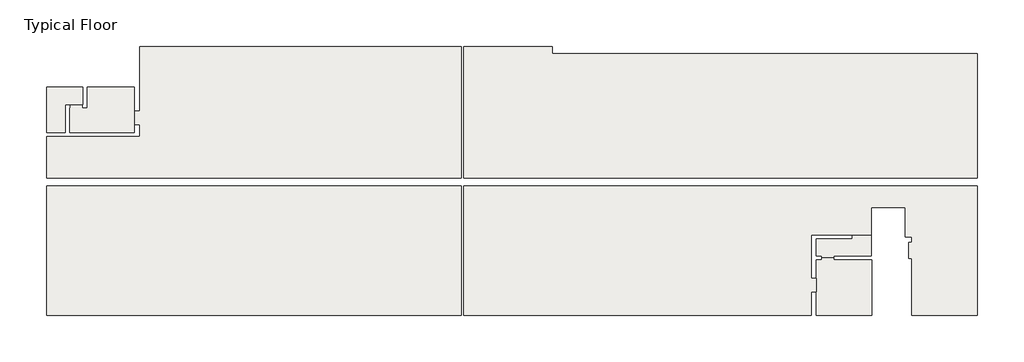
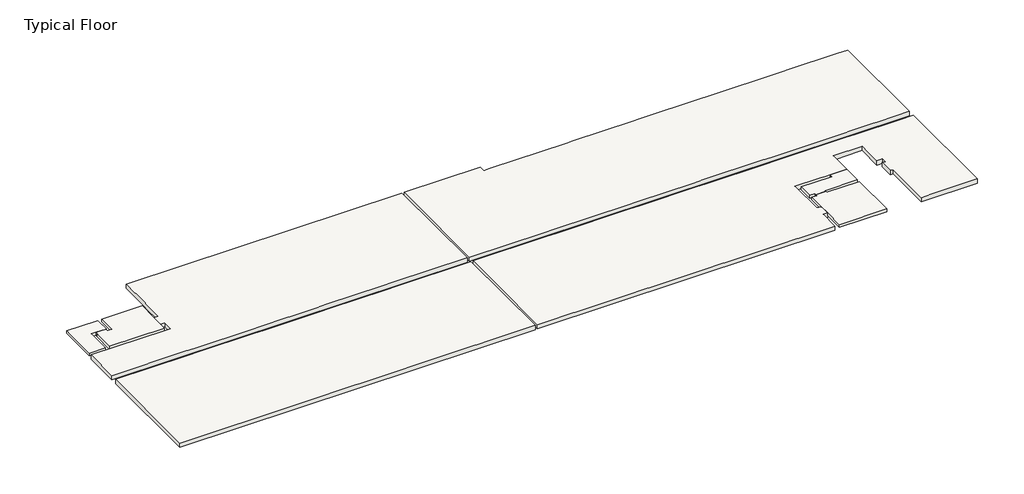
# One storey: 8 slabs.
"""IFC4 building model written with IfcOpenShell, lengths in millimetres."""

from ifc_helpers import new_model, si_unit, frame, origin, place, context, project, spatial, polyline, outline, extrude, faceted_brep, element, save

model = new_model("IFC4")

# Units and contexts
model_context = context("Model", 3, world=origin())
ifc_project = project(units=[si_unit("LENGTHUNIT", "METRE", prefix="MILLI")], contexts=[model_context])

# Site, building, storey
site = spatial("IfcSite", under=ifc_project)
building = spatial("IfcBuilding", under=site)
storey = spatial("IfcBuildingStorey", under=building, Name="Typical Floor", Elevation=4500.0)

# Slabs
placement = place(None, origin())
element("IfcSlab", 1, ObjectType="25", at=placement, inside=storey, context=model_context, shape_type="Brep", body=[
    faceted_brep([(22592.8106957, -3883.3566788, 4250.0), (23037.1054794, -3883.3566788, 4250.0), (23037.1054794, -3733.3566788, 4250.0), (23943.9406174, -3733.3566788, 4250.0), (23943.9406174, -3883.3566788, 4250.0), (26869.9357672, -3883.3566788, 4250.0), (26893.3884, -3883.3566788, 4250.0), (26893.3884, -8183.3289062, 4250.0), (22592.8106957, -8183.3289062, 4250.0), (22592.8106957, -6342.9498143, 4250.0), (23037.1054794, -3883.3566788, 4500.0), (22592.8106957, -3883.3566788, 4500.0), (22592.8106957, -5323.3186801, 4500.0), (22592.8106957, -6342.9498143, 4500.0), (22592.8106957, -8183.3289062, 4500.0), (26893.3884, -8183.3289062, 4500.0), (26893.3884, -3883.3566788, 4500.0), (26869.9357672, -3883.3566788, 4500.0), (23943.9406174, -3883.3566788, 4500.0), (23943.9406174, -3733.3566788, 4500.0), (23037.1054794, -3733.3566788, 4500.0)], [[[0, 1, 2, 3, 4, 5, 6, 7, 8, 9]], [[10, 11, 12, 13, 14, 15, 16, 17, 18, 19, 20]], [[1, 0, 11, 10]], [[2, 1, 10, 20]], [[3, 2, 20, 19]], [[4, 3, 19, 18]], [[4, 18, 17, 16, 6, 5]], [[7, 6, 16, 15]], [[8, 7, 15, 14]], [[9, 8, 14, 13]], [[0, 9, 13, 12, 11]]]),
])
element("IfcSlab", 2, ObjectType="25", at=placement, inside=storey, context=model_context, shape_type="SweptSolid", body=[
    extrude(outline(polyline([(26869.9357672, -1932.7380409), (26869.9357672, -3583.3566788), (23943.9406174, -3583.3566788), (23943.9406174, -3733.3566788), (23037.1054794, -3733.3566788), (23037.1054794, -3583.3566788), (22592.8106957, -3583.3566788), (22592.8106957, -2232.7380409), (25386.8359355, -2232.7380409), (25386.8359355, -1932.7380409), (26869.9357672, -1932.7380409)])), frame((0.0, 0.0, 4250.0), z_axis=(0.0, 0.0, 1.0), x_axis=(1.0, 0.0, 0.0)), (0.0, 0.0, 1.0), 250.0),
])
element("IfcSlab", 3, ObjectType="25", at=placement, inside=storey, context=model_context, shape_type="Brep", body=[
    faceted_brep([(-30180.4573498, 5997.6022486, 4250.0), (-35175.2356133, 5997.6022486, 4250.0), (-35175.2356133, 7897.529186, 4250.0), (-35131.0080225, 7897.529186, 4250.0), (-35131.0080225, 8167.529186, 4250.0), (-34230.8736368, 8167.529186, 4250.0), (-34230.8736368, 7897.529186, 4250.0), (-33829.9452937, 7897.529186, 4250.0), (-33829.9452937, 8167.529186, 4250.0), (-33829.9452937, 9500.978884, 4250.0), (-30180.4573498, 9500.978884, 4250.0), (-30180.4573498, 7652.6880547, 4250.0), (-30180.4573498, 6627.4729602, 4250.0), (-35175.2356133, 5997.6022486, 4500.0), (-30180.4573498, 5997.6022486, 4500.0), (-30180.4573498, 6627.4729602, 4500.0), (-30180.4573498, 7652.6880547, 4500.0), (-30180.4573498, 9500.978884, 4500.0), (-33829.9452937, 9500.978884, 4500.0), (-33829.9452937, 8167.529186, 4500.0), (-33829.9452937, 7897.529186, 4500.0), (-34230.8736368, 7897.529186, 4500.0), (-34230.8736368, 8167.529186, 4500.0), (-35131.0080225, 8167.529186, 4500.0), (-35131.0080225, 7897.529186, 4500.0), (-35175.2356133, 7897.529186, 4500.0)], [[[0, 1, 2, 3, 4, 5, 6, 7, 8, 9, 10, 11, 12]], [[13, 14, 15, 16, 17, 18, 19, 20, 21, 22, 23, 24, 25]], [[1, 0, 14, 13]], [[2, 1, 13, 25]], [[3, 2, 25, 24]], [[4, 3, 24, 23]], [[5, 4, 23, 22]], [[6, 5, 22, 21]], [[7, 6, 21, 20]], [[7, 20, 19, 18, 9, 8]], [[10, 9, 18, 17]], [[10, 17, 16, 15, 14, 0, 12, 11]]]),
])
element("IfcSlab", 4, ObjectType="25", at=placement, inside=storey, context=model_context, shape_type="Brep", body=[
    faceted_brep([(-36981.5324359, 5997.6022486, 4250.0), (-36981.5324359, 9500.978884, 4250.0), (-34179.9452937, 9500.978884, 4250.0), (-34179.9452937, 8167.529186, 4250.0), (-34230.8736368, 8167.529186, 4250.0), (-35131.0080225, 8167.529186, 4250.0), (-35525.2356133, 8167.529186, 4250.0), (-35525.2356133, 7897.529186, 4250.0), (-35525.2356133, 5997.6022486, 4250.0), (-36981.5324359, 9500.978884, 4500.0), (-36981.5324359, 5997.6022486, 4500.0), (-35525.2356133, 5997.6022486, 4500.0), (-35525.2356133, 7897.529186, 4500.0), (-35525.2356133, 8167.529186, 4500.0), (-35131.0080225, 8167.529186, 4500.0), (-34230.8736368, 8167.529186, 4500.0), (-34179.9452937, 8167.529186, 4500.0), (-34179.9452937, 9500.978884, 4500.0)], [[[0, 1, 2, 3, 4, 5, 6, 7, 8]], [[9, 10, 11, 12, 13, 14, 15, 16, 17]], [[1, 0, 10, 9]], [[2, 1, 9, 17]], [[3, 2, 17, 16]], [[3, 16, 15, 14, 13, 6, 5, 4]], [[6, 13, 12, 11, 8, 7]], [[0, 8, 11, 10]]]),
])
element("IfcSlab", 5, ObjectType="40", at=placement, inside=storey, context=model_context, shape_type="Brep", body=[
    faceted_brep([(-4686.1401685, 1852.6133039, 4100.0), (35073.6352373, 1852.6133039, 4100.0), (35073.6352373, -8183.3289062, 4100.0), (29994.7199004, -8183.3289062, 4100.0), (29994.7199004, -3766.5105737, 4100.0), (29744.7199004, -3766.5105737, 4100.0), (29744.7199004, -2514.5866947, 4100.0), (29994.7199004, -2514.5866947, 4100.0), (29994.7199004, -2110.3079756, 4100.0), (29744.7199004, -2110.3079756, 4100.0), (29495.5138576, -2110.3079756, 4100.0), (29495.5138576, 189.1668387, 4100.0), (29245.5138576, 189.1668387, 4100.0), (27139.9357672, 189.1668387, 4100.0), (26869.9357672, 189.1668387, 4100.0), (26869.9357672, -1932.7380409, 4100.0), (25386.8359355, -1932.7380409, 4100.0), (22592.8106957, -1932.7380409, 4100.0), (22192.8106957, -1932.7380409, 4100.0), (22192.8106957, -5323.3186801, 4100.0), (22592.8106957, -5323.3186801, 4100.0), (22592.8106957, -6342.9498143, 4100.0), (22192.8106957, -6342.9498143, 4100.0), (22192.8106957, -8183.3289062, 4100.0), (-4686.1401685, -8183.3289062, 4100.0), (35073.6352373, 1852.6133039, 4500.0), (34927.3208435, 1852.6133039, 4500.0), (34027.3208435, 1852.6133039, 4500.0), (29920.3049975, 1852.6133039, 4500.0), (29020.3049975, 1852.6133039, 4500.0), (22627.3114752, 1852.6133039, 4500.0), (21727.3114752, 1852.6133039, 4500.0), (16420.7293524, 1852.6133039, 4500.0), (15520.7293524, 1852.6133039, 4500.0), (10422.0355776, 1852.6133039, 4500.0), (9522.0355776, 1852.6133039, 4500.0), (2924.3455353, 1852.6133039, 4500.0), (2024.3455353, 1852.6133039, 4500.0), (-4686.1401685, 1852.6133039, 4500.0), (-4686.1401685, -8183.3289062, 4500.0), (22192.8106957, -8183.3289062, 4500.0), (22192.8106957, -6342.9498143, 4500.0), (22592.8106957, -6342.9498143, 4500.0), (22592.8106957, -5323.3186801, 4500.0), (22192.8106957, -5323.3186801, 4500.0), (22192.8106957, -1932.7380409, 4500.0), (22592.8106957, -1932.7380409, 4500.0), (25386.8359355, -1932.7380409, 4500.0), (26869.9357672, -1932.7380409, 4500.0), (26869.9357672, 189.1668387, 4500.0), (27139.9357672, 189.1668387, 4500.0), (29245.5138576, 189.1668387, 4500.0), (29495.5138576, 189.1668387, 4500.0), (29495.5138576, -2110.3079756, 4500.0), (29744.7199004, -2110.3079756, 4500.0), (29994.7199004, -2110.3079756, 4500.0), (29994.7199004, -2514.5866947, 4500.0), (29744.7199004, -2514.5866947, 4500.0), (29744.7199004, -3766.5105737, 4500.0), (29994.7199004, -3766.5105737, 4500.0), (29994.7199004, -8183.3289062, 4500.0), (30873.6352373, -8183.3289062, 4500.0), (35073.6352373, -8183.3289062, 4500.0), (26869.9357672, -1932.7380409, 4250.0), (25386.8359355, -1932.7380409, 4250.0), (22592.8106957, -5323.3186801, 4250.0), (22592.8106957, -6342.9498143, 4250.0)], [[[0, 1, 2, 3, 4, 5, 6, 7, 8, 9, 10, 11, 12, 13, 14, 15, 16, 17, 18, 19, 20, 21, 22, 23, 24]], [[25, 26, 27, 28, 29, 30, 31, 32, 33, 34, 35, 36, 37, 38, 39, 40, 41, 42, 43, 44, 45, 46, 47, 48, 49, 50, 51, 52, 53, 54, 55, 56, 57, 58, 59, 60, 61, 62]], [[1, 0, 38, 37, 36, 35, 34, 33, 32, 31, 30, 29, 28, 27, 26, 25]], [[2, 1, 25, 62]], [[3, 2, 62, 61, 60]], [[4, 3, 60, 59]], [[5, 4, 59, 58]], [[6, 5, 58, 57]], [[7, 6, 57, 56]], [[8, 7, 56, 55]], [[8, 55, 54, 53, 10, 9]], [[11, 10, 53, 52]], [[11, 52, 51, 50, 49, 14, 13, 12]], [[15, 14, 49, 48, 63]], [[16, 15, 63, 48, 47, 64]], [[45, 18, 17, 16, 64, 47, 46]], [[19, 18, 45, 44]], [[20, 19, 44, 43, 65]], [[21, 20, 65, 43, 42, 66]], [[22, 21, 66, 42, 41]], [[23, 22, 41, 40]], [[24, 23, 40, 39]], [[0, 24, 39, 38]]]),
])
element("IfcSlab", 6, ObjectType="40", at=placement, inside=storey, context=model_context, shape_type="Brep", body=[
    faceted_brep([(-4886.1401685, 1852.6133039, 4100.0), (-4886.1401685, -8183.3289062, 4100.0), (-36981.5324359, -8183.3289062, 4100.0), (-36981.5324359, 1852.6133039, 4100.0), (-4886.1401685, 1852.6133039, 4500.0), (-11589.7528998, 1852.6133039, 4500.0), (-12489.7528998, 1852.6133039, 4500.0), (-17591.3777818, 1852.6133039, 4500.0), (-18491.3777818, 1852.6133039, 4500.0), (-23534.5891488, 1852.6133039, 4500.0), (-24434.5891488, 1852.6133039, 4500.0), (-29484.6297539, 1852.6133039, 4500.0), (-30384.6297539, 1852.6133039, 4500.0), (-36981.5324359, 1852.6133039, 4500.0), (-36981.5324359, -8183.3289062, 4500.0), (-4886.1401685, -8183.3289062, 4500.0)], [[[0, 1, 2, 3]], [[4, 5, 6, 7, 8, 9, 10, 11, 12, 13, 14, 15]], [[1, 0, 4, 15]], [[2, 1, 15, 14]], [[3, 2, 14, 13]], [[0, 3, 13, 12, 11, 10, 9, 8, 7, 6, 5, 4]]]),
])
element("IfcSlab", 7, ObjectType="40", at=placement, inside=storey, context=model_context, shape_type="Brep", body=[
    faceted_brep([(2174.3455353, 12665.9833477, 4100.0), (2174.3455353, 12115.9833477, 4100.0), (2774.3455353, 12115.9833477, 4100.0), (9672.0355776, 12115.9833477, 4100.0), (10272.0355776, 12115.9833477, 4100.0), (15670.7293524, 12115.9833477, 4100.0), (16270.7293524, 12115.9833477, 4100.0), (21877.3114752, 12115.9833477, 4100.0), (22477.3114752, 12115.9833477, 4100.0), (29170.3049975, 12115.9833477, 4100.0), (29770.3049975, 12115.9833477, 4100.0), (34177.3208435, 12115.9833477, 4100.0), (34777.3208435, 12115.9833477, 4100.0), (35073.6352373, 12115.9833477, 4100.0), (35073.6352373, 2452.6133039, 4100.0), (-4686.1401685, 2452.6133039, 4100.0), (-4686.1401685, 12665.9833477, 4100.0), (2174.3455353, 12115.9833477, 4500.0), (2174.3455353, 12665.9833477, 4500.0), (-4686.1401685, 12665.9833477, 4500.0), (-4686.1401685, 2452.6133039, 4500.0), (2024.3455353, 2452.6133039, 4500.0), (2924.3455353, 2452.6133039, 4500.0), (9522.0355776, 2452.6133039, 4500.0), (10422.0355776, 2452.6133039, 4500.0), (15520.7293524, 2452.6133039, 4500.0), (16420.7293524, 2452.6133039, 4500.0), (21727.3114752, 2452.6133039, 4500.0), (22627.3114752, 2452.6133039, 4500.0), (29020.3049975, 2452.6133039, 4500.0), (29920.3049975, 2452.6133039, 4500.0), (34027.3208435, 2452.6133039, 4500.0), (34927.3208435, 2452.6133039, 4500.0), (35073.6352373, 2452.6133039, 4500.0), (35073.6352373, 12115.9833477, 4500.0), (34777.3208435, 12115.9833477, 4500.0), (34177.3208435, 12115.9833477, 4500.0), (29770.3049975, 12115.9833477, 4500.0), (29170.3049975, 12115.9833477, 4500.0), (22477.3114752, 12115.9833477, 4500.0), (21877.3114752, 12115.9833477, 4500.0), (16270.7293524, 12115.9833477, 4500.0), (15670.7293524, 12115.9833477, 4500.0), (10272.0355776, 12115.9833477, 4500.0), (9672.0355776, 12115.9833477, 4500.0), (2774.3455353, 12115.9833477, 4500.0)], [[[0, 1, 2, 3, 4, 5, 6, 7, 8, 9, 10, 11, 12, 13, 14, 15, 16]], [[17, 18, 19, 20, 21, 22, 23, 24, 25, 26, 27, 28, 29, 30, 31, 32, 33, 34, 35, 36, 37, 38, 39, 40, 41, 42, 43, 44, 45]], [[1, 0, 18, 17]], [[1, 17, 45, 44, 43, 42, 41, 40, 39, 38, 37, 36, 35, 34, 13, 12, 11, 10, 9, 8, 7, 6, 5, 4, 3, 2]], [[14, 13, 34, 33]], [[15, 14, 33, 32, 31, 30, 29, 28, 27, 26, 25, 24, 23, 22, 21, 20]], [[16, 15, 20, 19]], [[0, 16, 19, 18]]]),
])
element("IfcSlab", 8, ObjectType="40", at=placement, inside=storey, context=model_context, shape_type="Brep", body=[
    faceted_brep([(-29780.4573498, 5697.6022486, 4100.0), (-29780.4573498, 6627.4729602, 4100.0), (-30180.4573498, 6627.4729602, 4100.0), (-30180.4573498, 7652.6880547, 4100.0), (-29780.4573498, 7652.6880547, 4100.0), (-29780.4573498, 9500.978884, 4100.0), (-29780.4573498, 9800.978884, 4100.0), (-29780.4573498, 12665.9833477, 4100.0), (-4886.1401685, 12665.9833477, 4100.0), (-4886.1401685, 2452.6133039, 4100.0), (-36981.5324359, 2452.6133039, 4100.0), (-36981.5324359, 5697.6022486, 4100.0), (-30180.4573498, 5697.6022486, 4100.0), (-29780.4573498, 6627.4729602, 4500.0), (-29780.4573498, 5697.6022486, 4500.0), (-30180.4573498, 5697.6022486, 4500.0), (-36981.5324359, 5697.6022486, 4500.0), (-36981.5324359, 2452.6133039, 4500.0), (-30384.6297539, 2452.6133039, 4500.0), (-29484.6297539, 2452.6133039, 4500.0), (-24434.5891488, 2452.6133039, 4500.0), (-23534.5891488, 2452.6133039, 4500.0), (-18491.3777818, 2452.6133039, 4500.0), (-17591.3777818, 2452.6133039, 4500.0), (-12489.7528998, 2452.6133039, 4500.0), (-11589.7528998, 2452.6133039, 4500.0), (-4886.1401685, 2452.6133039, 4500.0), (-4886.1401685, 12665.9833477, 4500.0), (-29780.4573498, 12665.9833477, 4500.0), (-29780.4573498, 9800.978884, 4500.0), (-29780.4573498, 9500.978884, 4500.0), (-29780.4573498, 7652.6880547, 4500.0), (-30180.4573498, 7652.6880547, 4500.0), (-30180.4573498, 6627.4729602, 4500.0)], [[[0, 1, 2, 3, 4, 5, 6, 7, 8, 9, 10, 11, 12]], [[13, 14, 15, 16, 17, 18, 19, 20, 21, 22, 23, 24, 25, 26, 27, 28, 29, 30, 31, 32, 33]], [[14, 0, 12, 11, 16, 15]], [[1, 0, 14, 13]], [[8, 7, 28, 27]], [[9, 8, 27, 26]], [[10, 9, 26, 25, 24, 23, 22, 21, 20, 19, 18, 17]], [[11, 10, 17, 16]], [[2, 1, 13, 33]], [[3, 2, 33, 32]], [[4, 3, 32, 31]], [[4, 31, 30, 29, 28, 7, 6, 5]]]),
])

save(model, "model.ifc")

# Revit data of these elements
# Type "25"
#   Function = 0
#   Layers, outside or top first: 25 cm "Concrete" (function 1)
# Type "40"
#   Function = 0
#   Layers, outside or top first: 40 cm "Concrete" (function 1)
# Element 1 (IfcSlab, "25")
#   Mark = "S1"
#   SOFiSTiK_AMG_Comments = ""
#   built-in parameter 1001955 = 1.5708 (stored number, unit not read)
#   Height Offset From Level = 0 cm
#   built-in parameter 1001954 = 1
#   SOFiSTiK_AMG_Scheduled = yes
#   SOFiSTiK_AMG_Adjusted = yes
#   Phase Created = New Construction
#   Materials on its faces: "Concrete"
# Element 2 (IfcSlab, "25")
#   Mark = "S2"
#   SOFiSTiK_AMG_Comments = ""
#   Height Offset From Level = 0 cm
#   built-in parameter 1001954 = 1
#   SOFiSTiK_AMG_Scheduled = yes
#   SOFiSTiK_AMG_Adjusted = yes
#   Phase Created = New Construction
#   Materials on its faces: "Concrete"
# Element 3 (IfcSlab, "25")
#   Mark = "S3"
#   SOFiSTiK_AMG_Comments = ""
#   Height Offset From Level = 0 cm
#   built-in parameter 1001954 = 1
#   SOFiSTiK_AMG_Scheduled = yes
#   SOFiSTiK_AMG_Adjusted = yes
#   Phase Created = New Construction
#   Materials on its faces: "Concrete"
# Element 4 (IfcSlab, "25")
#   Mark = "S4"
#   SOFiSTiK_AMG_Comments = ""
#   built-in parameter 1001955 = 3.14159 (stored number, unit not read)
#   Height Offset From Level = 0 cm
#   built-in parameter 1001954 = 1
#   SOFiSTiK_AMG_Scheduled = yes
#   SOFiSTiK_AMG_Adjusted = yes
#   Phase Created = New Construction
#   Materials on its faces: "Concrete"
# Element 5 (IfcSlab, "40")
#   Mark = "S5"
#   SOFiSTiK_AMG_Comments = ""
#   built-in parameter 1001955 = 1.5708 (stored number, unit not read)
#   Height Offset From Level = 0 cm
#   built-in parameter 1001954 = 1
#   SOFiSTiK_AMG_Scheduled = yes
#   SOFiSTiK_AMG_Adjusted = yes
#   Phase Created = New Construction
#   Materials on its faces: "Concrete"
# Element 6 (IfcSlab, "40")
#   Mark = "S6"
#   SOFiSTiK_AMG_Comments = ""
#   Height Offset From Level = 0 cm
#   built-in parameter 1001954 = 1
#   SOFiSTiK_AMG_Scheduled = yes
#   SOFiSTiK_AMG_Adjusted = yes
#   Phase Created = New Construction
#   Materials on its faces: "Concrete"
# Element 7 (IfcSlab, "40")
#   Mark = "S7"
#   SOFiSTiK_AMG_Comments = ""
#   Height Offset From Level = 0 cm
#   built-in parameter 1001954 = 1
#   SOFiSTiK_AMG_Scheduled = yes
#   SOFiSTiK_AMG_Adjusted = yes
#   Phase Created = New Construction
#   Materials on its faces: "Concrete"
# Element 8 (IfcSlab, "40")
#   Mark = "S8"
#   SOFiSTiK_AMG_Comments = ""
#   built-in parameter 1001955 = 1.5708 (stored number, unit not read)
#   Height Offset From Level = 0 cm
#   built-in parameter 1001954 = 1
#   SOFiSTiK_AMG_Scheduled = yes
#   SOFiSTiK_AMG_Adjusted = yes
#   Phase Created = New Construction
#   Materials on its faces: "Concrete"
# Materials
#   "Concrete": class "Concrete", colour RGB 192 192 192, transparency 0, Keynote = "01000", Description = "Cast-in-place concrete", Cost = 0
